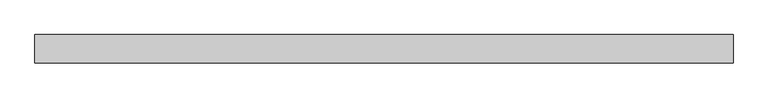
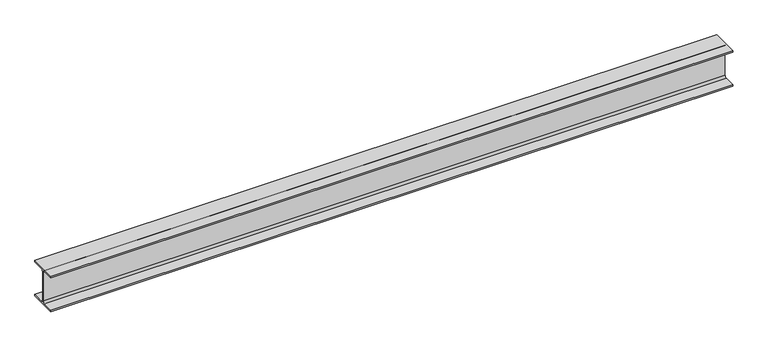
"""IFC4 building model written with IfcOpenShell, lengths in millimetres: beam geometry, 0912_Steel Framing_H-KSD3502 : H_SB_ASB_H-340x250x9x14."""

from ifc_helpers import new_model, si_unit, point, frame, frame_2d, origin, place, context, project, spatial, polyline, circle_curve, trimmed, segment, composite_curve, outline, extrude, source, transform, mapped, element, save


def beam_8c186262(model_context):
    return source(origin(), model_context, "Body", "SweptSolid", [
        extrude(outline(composite_curve([segment(polyline([(125.0, -156.0), (125.0, -170.0), (-125.0, -170.0), (-125.0, -156.0), (-24.5, -156.0)]), True, "CONTINUOUS"), segment(trimmed(circle_curve(frame_2d((-24.5, -136.0)), 20.0), [point((-24.5, -156.0))], [point((-4.5, -136.0))], True, "CARTESIAN"), True, "CONTINUOUS"), segment(polyline([(-4.5, -136.0), (-4.5, 136.0)]), True, "CONTINUOUS"), segment(trimmed(circle_curve(frame_2d((-24.5, 136.0)), 20.0), [point((-4.5, 136.0))], [point((-24.5, 156.0))], True, "CARTESIAN"), True, "CONTINUOUS"), segment(polyline([(-24.5, 156.0), (-125.0, 156.0), (-125.0, 170.0), (125.0, 170.0), (125.0, 156.0), (24.5, 156.0)]), True, "CONTINUOUS"), segment(trimmed(circle_curve(frame_2d((24.5, 136.0)), 20.0), [point((24.5, 156.0))], [point((4.5, 136.0))], True, "CARTESIAN"), True, "CONTINUOUS"), segment(polyline([(4.5, 136.0), (4.5, -136.0)]), True, "CONTINUOUS"), segment(trimmed(circle_curve(frame_2d((24.5, -136.0)), 20.0), [point((4.5, -136.0))], [point((24.5, -156.0))], True, "CARTESIAN"), True, "CONTINUOUS"), segment(polyline([(24.5, -156.0), (125.0, -156.0)]), True, "CONTINUOUS")], self_intersect=False)), frame((-3087.3, 0.0, 0.0), z_axis=(1.0, 0.0, 0.0), x_axis=(0.0, 1.0, 0.0)), (0.0, 0.0, 1.0), 6174.6),
    ])


if __name__ == "__main__":
    model = new_model("IFC4")
    model_context = context("Model", 3, world=origin())
    ifc_project = project(units=[si_unit("LENGTHUNIT", "METRE", prefix="MILLI")], contexts=[model_context])
    site = spatial("IfcSite", under=ifc_project)
    building = spatial("IfcBuilding", under=site)
    placement = place(None, origin())
    beam_shape = beam_8c186262(model_context)
    element("IfcBeam", 1, ObjectType="0912_Steel Framing_H-KSD3502 : H_SB_ASB_H-340x250x9x14", at=placement, inside=building, context=model_context, shape_type="MappedRepresentation", body=[
        mapped(beam_shape, transform((0.0, 0.0, 0.0), x_axis=(1.0, 0.0, 0.0), y_axis=(0.0, 1.0, 0.0), z_axis=(0.0, 0.0, 1.0))),
    ])
    save(model, "model.ifc")

# Revit data of these elements
# Type "0912_Steel Framing_H-KSD3502 : H_SB_ASB_H-340x250x9x14"
#   H_WM Code_1 = "S01AA002-00001 | Main Steel Structure Fabrication Work | Shelter/Building | Medium Steel - Standard (90KG/M>Weight≥30KG/M) | Material: (   )"
#   H_WM Code_2 = "S03AA028-00001 | Main Steel Structure Erection Work | Shelter/Building | Medium Steel (90KG/M>Weight≥30KG/M) | Material: (   )"
#   H_WM Code_3 = "S01AA010-00001 | Main Steel Structure Fabrication Work | Shelter/Building | Steel Painting/Coating | for Non-Fireproofed Steel Surface, Surface Preparation, Primer, Second & Final Coat | Material: (   )"
#   H_Q'ty Cal Type Tag = "SB-Q2"
#   Width = 25.0 cm
#   Web Thickness = 0.9 cm
#   Web Fillet = 2.0 cm
#   Warping Constant = 969000.0 cm⁶
#   W = 0
#   Torsional Moment of Inertia = 53.6551 cm⁴
#   Section Area = 101.5 cm²
#   Plastic Modulus weak axis = 447.0 cm³
#   Plastic Modulus strong axis = 1410.0 cm³
#   Perimeter = 1.63 m²/m
#   Nominal Weight = 79.70 kgf/m
#   Moment of Inertia weak axis = 3650.00 cm⁴
#   Moment of Inertia strong axis = 21700.00 cm⁴
#   Height = 34.0 cm
#   Flange Thickness = 1.4 cm
#   Elastic Modulus weak axis = 292.0 cm³
#   Elastic Modulus strong axis = 1280.0 cm³
#   Centroid Vertical = 17.0 cm
#   Centroid Horizontal = 12.5 cm
#   Ix = 217000000
#   Length [instance default] = 1.5240 m
#   Zx = 1410000
#   b = 0.2500 m
#   h = 0.3400 m
#   r = 0.0200 m
#   s = 0.0090 m
#   t = 0.0140 m
#   A = 0.01015 m²
#   Structural Material [instance default] = Steel, 45-345
#   Assembly Code = ""
# Element 1 (IfcBeam, "0912_Steel Framing_H-KSD3502 : H_SB_ASB_H-340x250x9x14")
#   Structural Material = none
# Materials
#   "Steel, 45-345": class "Metal", colour RGB 189 187 185, transparency 0, Description = "Steel 345 MPa", Cost = 0
